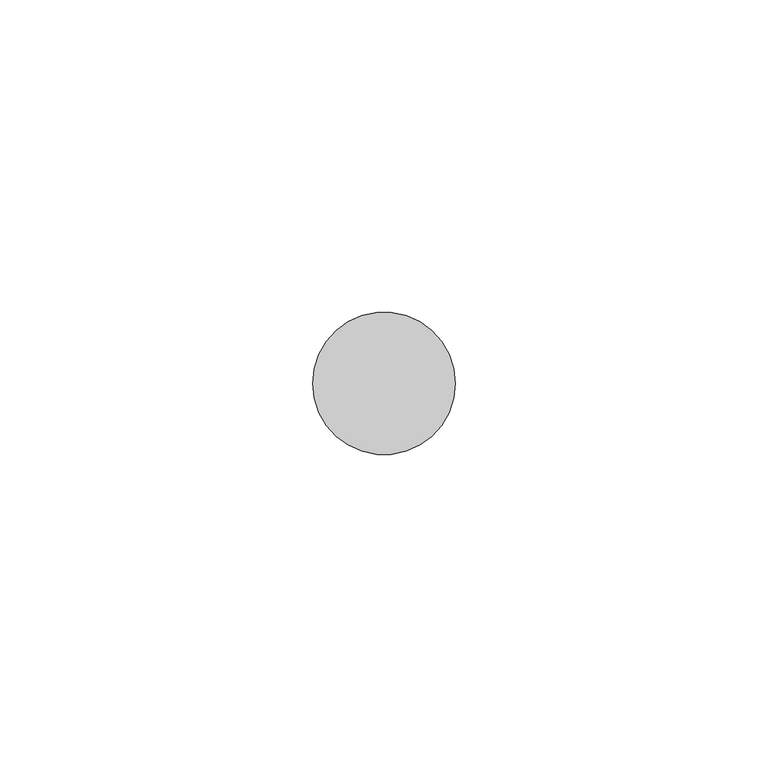
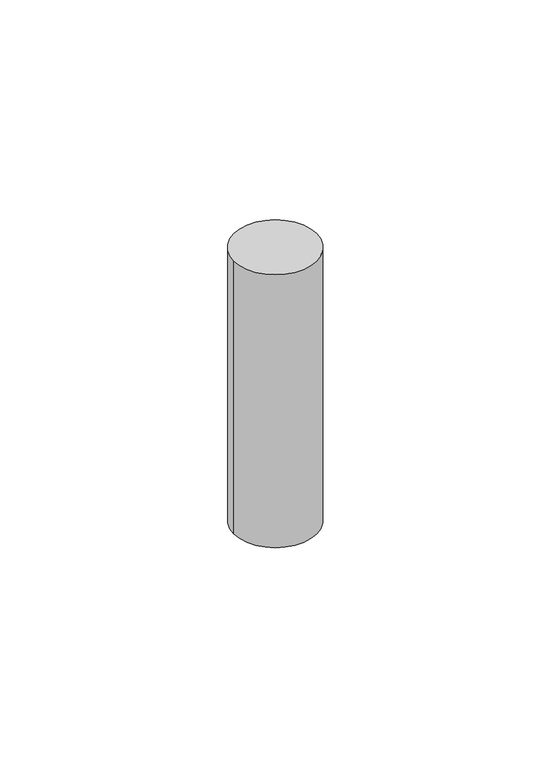
"""IFC4 building model written with IfcOpenShell, lengths in millimetres: proxy geometry, Bolt003 8693 : Bolt003 8693."""

from ifc_helpers import new_model, si_unit, point, frame, frame_2d, origin, place, context, project, spatial, circle_curve, trimmed, segment, composite_curve, outline, extrude, source, transform, mapped, element, save


def generic_models_a01074e3(model_context):
    return source(origin(), model_context, "Body", "SweptSolid", [
        extrude(outline(composite_curve([segment(trimmed(circle_curve(frame_2d((7415.2612305, -1781.8449707)), 11.4045168), [point((7403.8567137, -1781.8449707))], [point((7426.6657473, -1781.8449707))], False, "CARTESIAN"), True, "CONTINUOUS"), segment(trimmed(circle_curve(frame_2d((7415.2612305, -1781.8449707)), 11.4045168), [point((7426.6657473, -1781.8449707))], [point((7403.8567137, -1781.8449707))], False, "CARTESIAN"), True, "CONTINUOUS")], self_intersect=False)), frame((0.0, 0.0, 40049.196), z_axis=(0.0, 0.0, 1.0), x_axis=(1.0, 0.0, 0.0)), (0.0, 0.0, 1.0), 79.375),
    ])


if __name__ == "__main__":
    model = new_model("IFC4")
    model_context = context("Model", 3, world=origin())
    ifc_project = project(units=[si_unit("LENGTHUNIT", "METRE", prefix="MILLI")], contexts=[model_context])
    site = spatial("IfcSite", under=ifc_project)
    building = spatial("IfcBuilding", under=site)
    placement = place(None, origin())
    generic_models_shape = generic_models_a01074e3(model_context)
    element("IfcBuildingElementProxy", 1, Name="Bolt003 8693 : Bolt003 8693", ObjectType="Bolt003 8693 : Bolt003 8693", at=placement, inside=building, context=model_context, shape_type="MappedRepresentation", body=[
        mapped(generic_models_shape, transform((0.0, 0.0, 0.0), x_axis=(1.0, 0.0, 0.0), y_axis=(0.0, 1.0, 0.0), z_axis=(0.0, 0.0, 1.0))),
    ])
    save(model, "model.ifc")

# Revit data of these elements
# Type "Bolt003 8693 : Bolt003 8693"
#   NameOverride = "Bolt003"
# Element 1 (IfcBuildingElementProxy, "Bolt003 8693 : Bolt003 8693")
#   Materials on its faces: "BOLTS CONCEALED BY FLOOR FINISH"
# Materials
#   "BOLTS CONCEALED BY FLOOR FINISH": class "Unassigned", colour RGB 128 128 128, transparency 0
